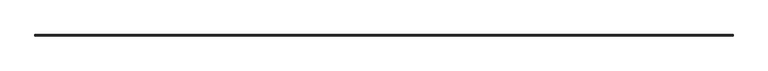
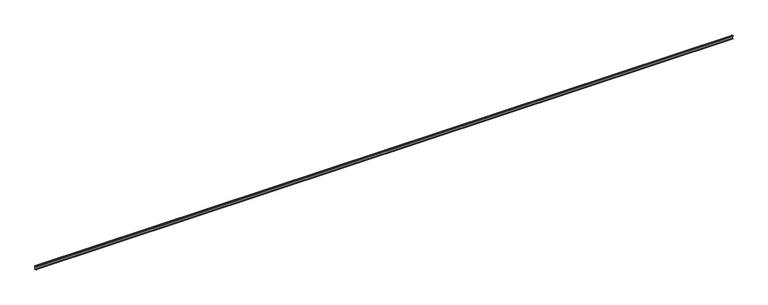
"""IFC4 building model written with IfcOpenShell, lengths in millimetres: beam geometry, 0912_Steel Framing_LC_KDS3530 : H_SB_AR_B03_LC-200x75x25x3.2."""

from ifc_helpers import new_model, si_unit, point, frame, frame_2d, origin, place, context, project, spatial, polyline, circle_curve, trimmed, segment, composite_curve, outline, extrude, source, transform, mapped, element, save


def beam_e488e9b8(model_context):
    return source(origin(), model_context, "Body", "SweptSolid", [
        extrude(outline(composite_curve([segment(polyline([(18.6, 87.5), (18.6, -87.5)]), True, "CONTINUOUS"), segment(trimmed(circle_curve(frame_2d((6.1, -87.5)), 12.5), [point((18.6, -87.5))], [point((6.1, -100.0))], False, "CARTESIAN"), True, "CONTINUOUS"), segment(polyline([(6.1, -100.0), (-43.9, -100.0)]), True, "CONTINUOUS"), segment(trimmed(circle_curve(frame_2d((-43.9, -87.5)), 12.5), [point((-43.9, -100.0))], [point((-56.4, -87.5))], False, "CARTESIAN"), True, "CONTINUOUS"), segment(polyline([(-56.4, -87.5), (-56.4, -75.0), (-51.9, -75.0), (-51.9, -87.5)]), True, "CONTINUOUS"), segment(trimmed(circle_curve(frame_2d((-43.9, -87.5)), 8.0), [point((-51.9, -87.5))], [point((-43.9, -95.5))], True, "CARTESIAN"), True, "CONTINUOUS"), segment(polyline([(-43.9, -95.5), (6.1, -95.5)]), True, "CONTINUOUS"), segment(trimmed(circle_curve(frame_2d((6.1, -87.5)), 8.0), [point((6.1, -95.5))], [point((14.1, -87.5))], True, "CARTESIAN"), True, "CONTINUOUS"), segment(polyline([(14.1, -87.5), (14.1, 87.5)]), True, "CONTINUOUS"), segment(trimmed(circle_curve(frame_2d((6.1, 87.5)), 8.0), [point((14.1, 87.5))], [point((6.1, 95.5))], True, "CARTESIAN"), True, "CONTINUOUS"), segment(polyline([(6.1, 95.5), (-41.1, 95.5)]), True, "CONTINUOUS"), segment(trimmed(circle_curve(frame_2d((-41.1, 87.5)), 8.0), [point((-41.1, 95.5))], [point((-49.1, 87.5))], True, "CARTESIAN"), True, "CONTINUOUS"), segment(polyline([(-49.1, 87.5), (-49.1, 75.0), (-53.6, 75.0), (-53.6, 87.5)]), True, "CONTINUOUS"), segment(trimmed(circle_curve(frame_2d((-41.1, 87.5)), 12.5), [point((-53.6, 87.5))], [point((-41.1, 100.0))], False, "CARTESIAN"), True, "CONTINUOUS"), segment(polyline([(-41.1, 100.0), (6.1, 100.0)]), True, "CONTINUOUS"), segment(trimmed(circle_curve(frame_2d((6.1, 87.5)), 12.5), [point((6.1, 100.0))], [point((18.6, 87.5))], False, "CARTESIAN"), True, "CONTINUOUS")], self_intersect=False)), frame((-19850.0, 0.0, 0.0), z_axis=(1.0, 0.0, 0.0), x_axis=(0.0, 1.0, 0.0)), (0.0, 0.0, 1.0), 39700.0),
    ])


if __name__ == "__main__":
    model = new_model("IFC4")
    model_context = context("Model", 3, world=origin())
    ifc_project = project(units=[si_unit("LENGTHUNIT", "METRE", prefix="MILLI")], contexts=[model_context])
    site = spatial("IfcSite", under=ifc_project)
    building = spatial("IfcBuilding", under=site)
    placement = place(None, origin())
    beam_shape = beam_e488e9b8(model_context)
    element("IfcBeam", 1, ObjectType="0912_Steel Framing_LC_KDS3530 : H_SB_AR_B03_LC-200x75x25x3.2", at=placement, inside=building, context=model_context, shape_type="MappedRepresentation", body=[
        mapped(beam_shape, transform((0.0, 0.0, 0.0), x_axis=(1.0, 0.0, 0.0), y_axis=(0.0, 1.0, 0.0), z_axis=(0.0, 0.0, 1.0))),
    ])
    save(model, "model.ifc")

# Revit data of these elements
# Type "0912_Steel Framing_LC_KDS3530 : H_SB_AR_B03_LC-200x75x25x3.2"
#   r = 8 mm
#   d = 25 mm
#   R = 11.2 mm
#   Perimeter = 0.78 m²/m
#   Nominal Weight = 14.00 kgf/m
#   Length [instance default] = 1000 mm
#   B = 75 mm
#   H = 200 mm
#   tw = 3.2 mm
#   x = 18.6 mm
#   A = 1.00 m²
#   Structural Material [instance default] = Steel, 45-345
#   Assembly Code = ""
# Element 1 (IfcBeam, "0912_Steel Framing_LC_KDS3530 : H_SB_AR_B03_LC-200x75x25x3.2")
#   Materials on its faces: "Steel, 45-345"
# Materials
#   "Steel, 45-345": class "Metal", colour RGB 189 187 185, transparency 0, Description = "Steel 345 MPa", Cost = 0
